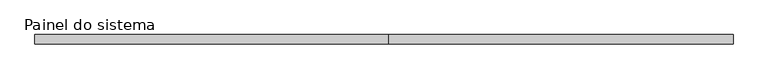
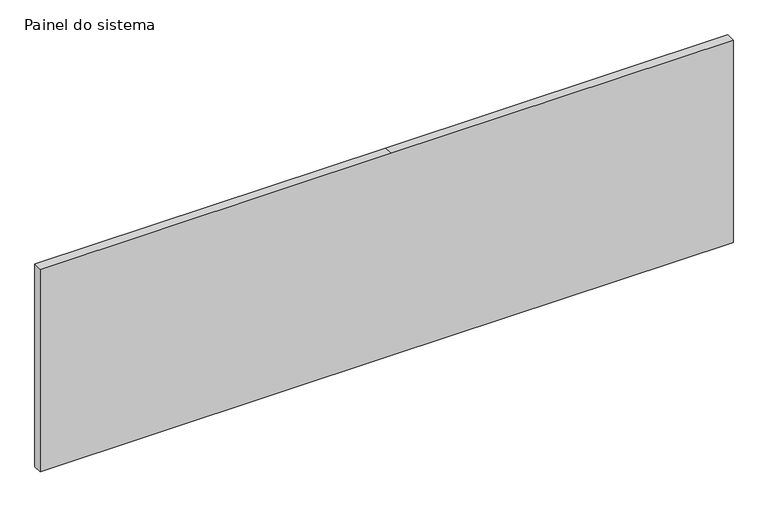
"""IFC4 building model written with IfcOpenShell, lengths in millimetres: plate geometry, Painel do sistema : Envidraçado."""

from ifc_helpers import new_model, si_unit, frame, origin, place, context, project, spatial, polyline, outline, extrude, source, transform, mapped, element, save


def painel_do_sistema_1f2b63a2(model_context):
    return source(origin(), model_context, "Body", "SweptSolid", [
        extrude(outline(polyline([(0.0, -954.2100001), (0.0, 12.4999998), (0.0, 954.2100001), (590.0, 954.2100001), (590.0, 12.4999998), (590.0, -954.2100001), (0.0, -954.2100001)])), frame((0.0, -49.5, 0.0), z_axis=(0.0, 1.0, 0.0), x_axis=(0.0, 0.0, 1.0)), (0.0, 0.0, 1.0), 25.0),
    ])


if __name__ == "__main__":
    model = new_model("IFC4")
    model_context = context("Model", 3, world=origin())
    ifc_project = project(units=[si_unit("LENGTHUNIT", "METRE", prefix="MILLI")], contexts=[model_context])
    site = spatial("IfcSite", under=ifc_project)
    building = spatial("IfcBuilding", under=site)
    placement = place(None, origin())
    painel_do_sistema_shape = painel_do_sistema_1f2b63a2(model_context)
    element("IfcPlate", 1, ObjectType="Painel do sistema : Envidraçado", at=placement, inside=building, context=model_context, shape_type="MappedRepresentation", body=[
        mapped(painel_do_sistema_shape, transform((0.0, 0.0, 0.0), x_axis=(1.0, 0.0, 0.0), y_axis=(0.0, 1.0, 0.0), z_axis=(0.0, 0.0, 1.0))),
    ])
    save(model, "model.ifc")

# Revit data of these elements
# Type "Painel do sistema : Envidraçado"
#   Construction Type Id = "GSP4R"
#   Analytic Construction = "Vidraça única Pilkington 1/8 pol"
#   Visual Light Transmittance = 0.9
#   Solar Heat Gain Coefficient = 0.86
#   Heat Transfer Coefficient (U) = 6.7069 W/(m²·K)
# Element 1 (IfcPlate, "Painel do sistema : Envidraçado")
#   Materials on its faces: ".VIDRO GENÉRICO"
# Materials
#   ".VIDRO GENÉRICO": class ".CC_VIDRO", colour RGB 0 128 192, transparency 0.9, Description = "Vidro comum", Cost = 0
